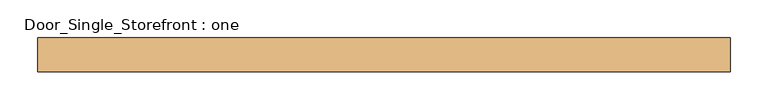
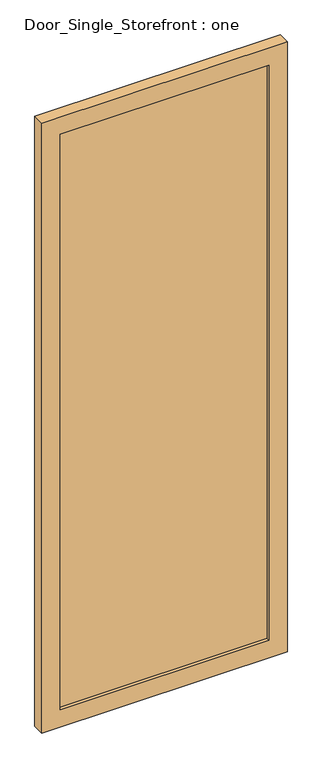
"""IFC4 building model written with IfcOpenShell, lengths in millimetres: door geometry, Door_Single_Storefront : one."""

from ifc_helpers import new_model, si_unit, frame, origin, place, context, project, spatial, polyline, outline, extrude, source, transform, mapped, element, save


def door_single_storefront_one_2a3449f9(model_context):
    return source(origin(), model_context, "Body", "SweptSolid", [
        extrude(outline(polyline([(388.9375, -6.35), (-388.9375, -6.35), (-388.9375, 12.7), (388.9375, 12.7), (388.9375, -6.35)])), frame((0.0, 0.0, 68.2625), z_axis=(0.0, 0.0, 1.0), x_axis=(1.0, 0.0, 0.0)), (0.0, 0.0, 1.0), 2263.3107725),
        extrude(outline(polyline([(2399.8357725, -457.2), (0.0, -457.2), (0.0, 457.2), (2399.8357725, 457.2), (2399.8357725, -457.2)]), holes=[polyline([(68.2625, 388.9375), (68.2625, -388.9375), (2331.5732725, -388.9375), (2331.5732725, 388.9375), (68.2625, 388.9375)])]), frame((0.0, -19.05, 0.0), z_axis=(0.0, 1.0, 0.0), x_axis=(0.0, 0.0, 1.0)), (0.0, 0.0, 1.0), 44.45),
    ])


if __name__ == "__main__":
    model = new_model("IFC4")
    model_context = context("Model", 3, world=origin())
    ifc_project = project(units=[si_unit("LENGTHUNIT", "METRE", prefix="MILLI")], contexts=[model_context])
    site = spatial("IfcSite", under=ifc_project)
    building = spatial("IfcBuilding", under=site)
    placement = place(None, origin())
    door_single_storefront_one_shape = door_single_storefront_one_2a3449f9(model_context)
    element("IfcDoor", 1, ObjectType="Door_Single_Storefront : one", at=placement, inside=building, context=model_context, shape_type="MappedRepresentation", body=[
        mapped(door_single_storefront_one_shape, transform((0.0, 0.0, 0.0), x_axis=(1.0, 0.0, 0.0), y_axis=(0.0, 1.0, 0.0), z_axis=(0.0, 0.0, 1.0))),
    ])
    save(model, "model.ifc")

# Revit data of these elements
# Type "Door_Single_Storefront : one"
#   Type Mark = "29"
#   OD_DS_Door_Material = "ALUM./GLAZING"
#   OD_DS_Door_Type = "STOREFRONT (NARROW STILE)"
#   OD_DS_Lockset = "ENTRY LOCK (INSIDE ADA LEVER ALWAYS ACTIVE)"
#   Analytic Construction = "<None>"
#   angle open [instance default] = 132.952°
#   Stile_Width = 0' - 2 11/16"
#   Door_Thickness = 0' - 1 3/4"
#   Door_Offset = 0' - 1"
#   Glass_Material = TEMPERED INSULATED GLAZING (CARDINAL GLASS LoĒ²-240\nOR EQUIVALENT)
#   Frame_Material = KAWNEER 260 INSULCLADTM THERMAL ENTRANCE - CLEAR ANODIZED ALUM.
#   Function = (empty or 0)
# Element 1 (IfcDoor, "Door_Single_Storefront : one")
#   Materials on its faces: "KAWNEER 260 INSULCLADTM THERMAL ENTRANCE - CLEAR ANODIZED ALUM.", "TEMPERED INSULATED GLAZING (CARDINAL GLASS LoĒ²-240\nOR EQUIVALENT)"
# Materials
#   "TEMPERED INSULATED GLAZING (CARDINAL GLASS LoĒ²-240\nOR EQUIVALENT)": class "Glass", colour RGB 196 205 210, transparency 0.85, Description = "Soda Lime Glass", Cost = 0
#   "KAWNEER 260 INSULCLADTM THERMAL ENTRANCE - CLEAR ANODIZED ALUM.": class "Metal", colour RGB 244 244 244, transparency 0, Description = "Aluminum 6061", Cost = 0
